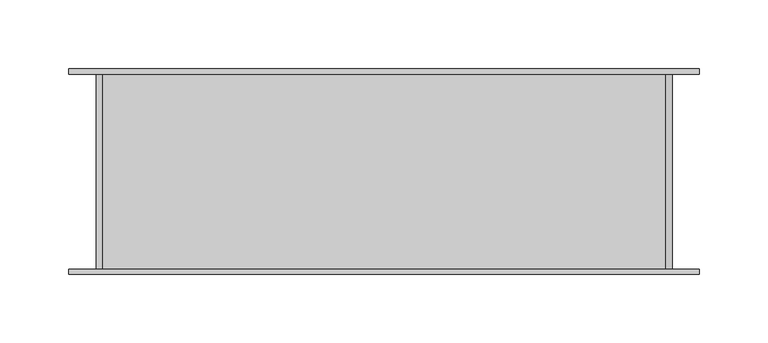
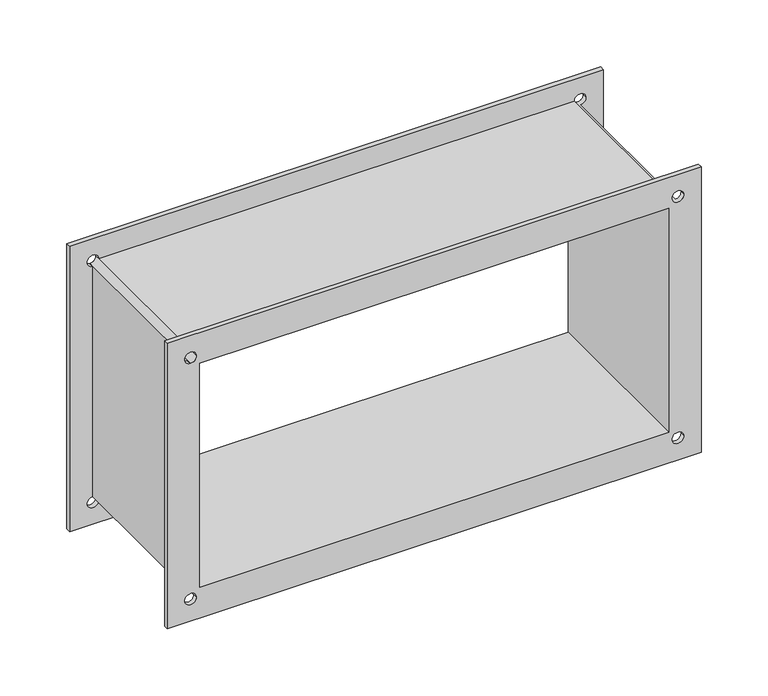
"""IFC4 building model written with IfcOpenShell, lengths in millimetres: proxy geometry, Гибкая вставка В : В 40-20."""

from ifc_helpers import new_model, si_unit, frame, origin, place, context, project, spatial, polyline, circle_curve, source, transform, mapped, element, save
from ifc_brep_helpers import plane_surface, revolved_surface, advanced_brep


def mechanical_equipment_3e9e5508(model_context):
    return source(origin(), model_context, "Body", "AdvancedBrep", [
        advanced_brep(
        [(230.0, 75.0, 130.0), (-230.0, 75.0, 130.0), (-230.0, 70.7949347, 130.0), (230.0, 70.7949347, 130.0), (-230.0, -75.0, 130.0), (230.0, -75.0, 130.0), (230.0, -71.2050653, 130.0), (-230.0, -71.2050653, 130.0), (230.0, -75.0, -130.0), (-230.0, -75.0, -130.0), (-230.0, -71.2050653, -130.0), (230.0, -71.2050653, -130.0), (-230.0, 75.0, -130.0), (230.0, 75.0, -130.0), (230.0, 70.7949347, -130.0), (-230.0, 70.7949347, -130.0), (202.0, 75.0, 102.0), (-202.0, 75.0, 102.0), (-202.0, 75.0, -102.0), (202.0, 75.0, -102.0), (-215.0, 75.0, 110.0), (-205.0, 75.0, 110.0), (205.0, 75.0, 110.0), (215.0, 75.0, 110.0), (205.0, 75.0, -110.0), (215.0, 75.0, -110.0), (-215.0, 75.0, -110.0), (-205.0, 75.0, -110.0), (-202.0, -75.0, 102.0), (202.0, -75.0, 102.0), (202.0, -75.0, -102.0), (-202.0, -75.0, -102.0), (-205.0, -75.0, 110.0), (-215.0, -75.0, 110.0), (215.0, -75.0, 110.0), (205.0, -75.0, 110.0), (215.0, -75.0, -110.0), (205.0, -75.0, -110.0), (-205.0, -75.0, -110.0), (-215.0, -75.0, -110.0), (210.0, 70.7949347, 105.0), (210.0, 70.7949347, -105.0), (215.0, 70.7949347, -110.0), (205.0, 70.7949347, -110.0), (-205.0, 70.7949347, -110.0), (-215.0, 70.7949347, -110.0), (-210.0, 70.7949347, -105.0), (-210.0, 70.7949347, 105.0), (-215.0, 70.7949347, 110.0), (-205.0, 70.7949347, 110.0), (205.0, 70.7949347, 110.0), (215.0, 70.7949347, 110.0), (210.0, -71.2050653, -105.0), (210.0, -71.2050653, 105.0), (215.0, -71.2050653, 110.0), (205.0, -71.2050653, 110.0), (-205.0, -71.2050653, 110.0), (-215.0, -71.2050653, 110.0), (-210.0, -71.2050653, 105.0), (-210.0, -71.2050653, -105.0), (-215.0, -71.2050653, -110.0), (-205.0, -71.2050653, -110.0), (205.0, -71.2050653, -110.0), (215.0, -71.2050653, -110.0)],
        [
            (0, 1),
            (1, 2),
            (2, 3),
            (3, 0),
            (4, 5),
            (5, 6),
            (6, 7),
            (7, 4),
            (8, 9),
            (9, 10),
            (10, 11),
            (11, 8),
            (12, 13),
            (13, 14),
            (14, 15),
            (15, 12),
            (0, 13),
            (12, 1),
            (16, 17),
            (17, 18),
            (18, 19),
            (19, 16),
            (20, 21, circle_curve(frame((-210.0, 75.0, 110.0), z_axis=(0.0, -1.0, 0.0), x_axis=(1.0, 0.0, 0.0)), 5.0)),
            (21, 20, circle_curve(frame((-210.0, 75.0, 110.0), z_axis=(0.0, -1.0, 0.0), x_axis=(1.0, 0.0, 0.0)), 5.0)),
            (22, 23, circle_curve(frame((210.0, 75.0, 110.0), z_axis=(0.0, -1.0, 0.0), x_axis=(1.0, 0.0, 0.0)), 5.0)),
            (23, 22, circle_curve(frame((210.0, 75.0, 110.0), z_axis=(0.0, -1.0, 0.0), x_axis=(1.0, 0.0, 0.0)), 5.0)),
            (24, 25, circle_curve(frame((210.0, 75.0, -110.0), z_axis=(0.0, -1.0, 0.0), x_axis=(1.0, 0.0, 0.0)), 5.0)),
            (25, 24, circle_curve(frame((210.0, 75.0, -110.0), z_axis=(0.0, -1.0, 0.0), x_axis=(1.0, 0.0, 0.0)), 5.0)),
            (26, 27, circle_curve(frame((-210.0, 75.0, -110.0), z_axis=(0.0, -1.0, 0.0), x_axis=(1.0, 0.0, 0.0)), 5.0)),
            (27, 26, circle_curve(frame((-210.0, 75.0, -110.0), z_axis=(0.0, -1.0, 0.0), x_axis=(1.0, 0.0, 0.0)), 5.0)),
            (15, 2),
            (9, 4),
            (7, 10),
            (8, 5),
            (28, 29),
            (29, 30),
            (30, 31),
            (31, 28),
            (32, 33, circle_curve(frame((-210.0, -75.0, 110.0), z_axis=(0.0, 1.0, 0.0), x_axis=(1.0, 0.0, 0.0)), 5.0)),
            (33, 32, circle_curve(frame((-210.0, -75.0, 110.0), z_axis=(0.0, 1.0, 0.0), x_axis=(1.0, 0.0, 0.0)), 5.0)),
            (34, 35, circle_curve(frame((210.0, -75.0, 110.0), z_axis=(0.0, 1.0, 0.0), x_axis=(1.0, 0.0, 0.0)), 5.0)),
            (35, 34, circle_curve(frame((210.0, -75.0, 110.0), z_axis=(0.0, 1.0, 0.0), x_axis=(1.0, 0.0, 0.0)), 5.0)),
            (36, 37, circle_curve(frame((210.0, -75.0, -110.0), z_axis=(0.0, 1.0, 0.0), x_axis=(1.0, 0.0, 0.0)), 5.0)),
            (37, 36, circle_curve(frame((210.0, -75.0, -110.0), z_axis=(0.0, 1.0, 0.0), x_axis=(1.0, 0.0, 0.0)), 5.0)),
            (38, 39, circle_curve(frame((-210.0, -75.0, -110.0), z_axis=(0.0, 1.0, 0.0), x_axis=(1.0, 0.0, 0.0)), 5.0)),
            (39, 38, circle_curve(frame((-210.0, -75.0, -110.0), z_axis=(0.0, 1.0, 0.0), x_axis=(1.0, 0.0, 0.0)), 5.0)),
            (3, 14),
            (11, 6),
            (28, 17),
            (16, 29),
            (31, 18),
            (30, 19),
            (40, 41),
            (41, 42, circle_curve(frame((210.0, 70.7949347, -110.0), z_axis=(0.0, 1.0, 0.0), x_axis=(1.0, 0.0, 0.0)), 5.0)),
            (42, 43, circle_curve(frame((210.0, 70.7949347, -110.0), z_axis=(0.0, 1.0, 0.0), x_axis=(1.0, 0.0, 0.0)), 5.0)),
            (43, 44),
            (44, 45, circle_curve(frame((-210.0, 70.7949347, -110.0), z_axis=(0.0, 1.0, 0.0), x_axis=(1.0, 0.0, 0.0)), 5.0)),
            (45, 46, circle_curve(frame((-210.0, 70.7949347, -110.0), z_axis=(0.0, 1.0, 0.0), x_axis=(1.0, 0.0, 0.0)), 5.0)),
            (46, 47),
            (47, 48, circle_curve(frame((-210.0, 70.7949347, 110.0), z_axis=(0.0, 1.0, 0.0), x_axis=(1.0, 0.0, 0.0)), 5.0)),
            (48, 49, circle_curve(frame((-210.0, 70.7949347, 110.0), z_axis=(0.0, 1.0, 0.0), x_axis=(1.0, 0.0, 0.0)), 5.0)),
            (49, 50),
            (50, 51, circle_curve(frame((210.0, 70.7949347, 110.0), z_axis=(0.0, 1.0, 0.0), x_axis=(1.0, 0.0, 0.0)), 5.0)),
            (51, 40, circle_curve(frame((210.0, 70.7949347, 110.0), z_axis=(0.0, 1.0, 0.0), x_axis=(1.0, 0.0, 0.0)), 5.0)),
            (52, 53),
            (53, 54, circle_curve(frame((210.0, -71.2050653, 110.0), z_axis=(0.0, -1.0, 0.0), x_axis=(1.0, 0.0, 0.0)), 5.0)),
            (54, 55, circle_curve(frame((210.0, -71.2050653, 110.0), z_axis=(0.0, -1.0, 0.0), x_axis=(1.0, 0.0, 0.0)), 5.0)),
            (55, 56),
            (56, 57, circle_curve(frame((-210.0, -71.2050653, 110.0), z_axis=(0.0, -1.0, 0.0), x_axis=(1.0, 0.0, 0.0)), 5.0)),
            (57, 58, circle_curve(frame((-210.0, -71.2050653, 110.0), z_axis=(0.0, -1.0, 0.0), x_axis=(1.0, 0.0, 0.0)), 5.0)),
            (58, 59),
            (59, 60, circle_curve(frame((-210.0, -71.2050653, -110.0), z_axis=(0.0, -1.0, 0.0), x_axis=(1.0, 0.0, 0.0)), 5.0)),
            (60, 61, circle_curve(frame((-210.0, -71.2050653, -110.0), z_axis=(0.0, -1.0, 0.0), x_axis=(1.0, 0.0, 0.0)), 5.0)),
            (61, 62),
            (62, 63, circle_curve(frame((210.0, -71.2050653, -110.0), z_axis=(0.0, -1.0, 0.0), x_axis=(1.0, 0.0, 0.0)), 5.0)),
            (63, 52, circle_curve(frame((210.0, -71.2050653, -110.0), z_axis=(0.0, -1.0, 0.0), x_axis=(1.0, 0.0, 0.0)), 5.0)),
            (32, 56),
            (56, 49),
            (49, 21),
            (20, 48),
            (47, 58),
            (57, 33),
            (55, 35),
            (34, 54),
            (53, 40),
            (51, 23),
            (22, 50),
            (50, 55),
            (62, 37),
            (36, 63),
            (24, 43),
            (42, 25),
            (62, 43),
            (41, 52),
            (38, 61),
            (60, 39),
            (44, 27),
            (26, 45),
            (59, 46),
            (44, 61),
        ],
        [
            plane_surface(frame((-230.0, 75.0, 130.0), z_axis=(0.0, 0.0, 1.0), x_axis=(-1.0, 0.0, 0.0))),
            plane_surface(frame((-230.0, 75.0, -130.0), z_axis=(0.0, 0.0, -1.0), x_axis=(1.0, 0.0, 0.0))),
            plane_surface(frame((230.0, 75.0, 130.0), z_axis=(0.0, 1.0, 0.0), x_axis=(0.0, 0.0, -1.0))),
            plane_surface(frame((-230.0, 75.0, 130.0), z_axis=(-1.0, 0.0, 0.0), x_axis=(0.0, 0.0, -1.0))),
            plane_surface(frame((-230.0, -75.0, 130.0), z_axis=(0.0, -1.0, 0.0), x_axis=(0.0, 0.0, -1.0))),
            plane_surface(frame((230.0, -75.0, 130.0), z_axis=(1.0, 0.0, 0.0), x_axis=(0.0, 0.0, -1.0))),
            plane_surface(frame((202.0, -75.0, 102.0), z_axis=(0.0, 0.0, -1.0), x_axis=(0.0, 1.0, 0.0))),
            plane_surface(frame((-202.0, -75.0, 102.0), z_axis=(1.0, 0.0, 0.0), x_axis=(0.0, 1.0, 0.0))),
            plane_surface(frame((-202.0, -75.0, -102.0), z_axis=(0.0, 0.0, 1.0), x_axis=(0.0, 1.0, 0.0))),
            plane_surface(frame((202.0, -75.0, -102.0), z_axis=(-1.0, 0.0, 0.0), x_axis=(0.0, 1.0, 0.0))),
            plane_surface(frame((-230.0, 70.7949347, 130.0), z_axis=(0.0, -1.0, 0.0), x_axis=(1.0, 0.0, 0.0))),
            plane_surface(frame((-210.0, -71.2050653, 110.0), z_axis=(0.0, 1.0, 0.0), x_axis=(1.0, 0.0, 0.0))),
            revolved_surface(polyline([(-205.0, -75.0, 110.0), (-205.0, 75.0, 110.0)]), (-210.0, 75.0, 110.0), (0.0, -1.0, 0.0)),
            revolved_surface(polyline([(-205.0, -75.0, 110.0), (-205.0, -71.2050653, 110.0)]), (-210.0, 75.0, 110.0), (0.0, -1.0, 0.0)),
            revolved_surface(polyline([(-205.0, 70.7949347, 110.0), (-205.0, 75.0, 110.0)]), (-210.0, 75.0, 110.0), (0.0, -1.0, 0.0)),
            revolved_surface(polyline([(215.0, -75.0, 110.0), (215.0, 75.0, 110.0)]), (210.0, 0.0, 110.0), (0.0, -1.0, 0.0)),
            revolved_surface(polyline([(215.0, -75.0, 110.0), (215.0, -71.2050653, 110.0)]), (210.0, 0.0, 110.0), (0.0, -1.0, 0.0)),
            revolved_surface(polyline([(215.0, 70.7949347, 110.0), (215.0, 75.0, 110.0)]), (210.0, 0.0, 110.0), (0.0, -1.0, 0.0)),
            revolved_surface(polyline([(215.0, -75.0, -110.0), (215.0, -71.2050653, -110.0)]), (210.0, 0.0, -110.0), (0.0, -1.0, 0.0)),
            revolved_surface(polyline([(215.0, 70.7949347, -110.0), (215.0, 75.0, -110.0)]), (210.0, 0.0, -110.0), (0.0, -1.0, 0.0)),
            revolved_surface(polyline([(215.0, -75.0, -110.0), (215.0, 75.0, -110.0)]), (210.0, 0.0, -110.0), (0.0, -1.0, 0.0)),
            revolved_surface(polyline([(-205.0, -75.0, -110.0), (-205.0, -71.2050653, -110.0)]), (-210.0, 0.0, -110.0), (0.0, -1.0, 0.0)),
            revolved_surface(polyline([(-205.0, 70.7949347, -110.0), (-205.0, 75.0, -110.0)]), (-210.0, 0.0, -110.0), (0.0, -1.0, 0.0)),
            revolved_surface(polyline([(-205.0, -75.0, -110.0), (-205.0, 75.0, -110.0)]), (-210.0, 0.0, -110.0), (0.0, -1.0, 0.0)),
            plane_surface(frame((210.0, 70.7949347, 110.0), z_axis=(1.0, 0.0, 0.0), x_axis=(0.0, 0.0, -1.0))),
            plane_surface(frame((210.0, 70.7949347, -110.0), z_axis=(0.0, 0.0, -1.0), x_axis=(-1.0, 0.0, 0.0))),
            plane_surface(frame((-210.0, 70.7949347, -110.0), z_axis=(-1.0, 0.0, 0.0), x_axis=(0.0, 0.0, 1.0))),
            plane_surface(frame((-210.0, 70.7949347, 110.0), z_axis=(0.0, 0.0, 1.0), x_axis=(1.0, 0.0, 0.0))),
        ],
        [
            (0, [[1, 2, 3, 4]]),
            (0, [[5, 6, 7, 8]]),
            (1, [[9, 10, 11, 12]]),
            (1, [[13, 14, 15, 16]]),
            (2, [[-1, 17, -13, 18], [19, 20, 21, 22], [23, 24], [25, 26], [27, 28], [29, 30]]),
            (3, [[-18, -16, 31, -2]]),
            (3, [[32, -8, 33, -10]]),
            (4, [[-5, -32, -9, 34], [35, 36, 37, 38], [39, 40], [41, 42], [43, 44], [45, 46]]),
            (5, [[-17, -4, 47, -14]]),
            (5, [[-34, -12, 48, -6]]),
            (6, [[49, -19, 50, -35]]),
            (7, [[-49, -38, 51, -20]]),
            (8, [[-51, -37, 52, -21]]),
            (9, [[-50, -22, -52, -36]]),
            (10, [[-3, -31, -15, -47], [53, 54, 55, 56, 57, 58, 59, 60, 61, 62, 63, 64]]),
            (11, [[-7, -48, -11, -33], [65, 66, 67, 68, 69, 70, 71, 72, 73, 74, 75, 76]]),
            (12, [[77, 78, 79, -23, 80, -60, 81, -70, 82, -39]]),
            (13, [[-77, -40, -82, -69]]),
            (14, [[-79, -61, -80, -24]]),
            (15, [[83, -41, 84, -66, 85, -64, 86, -25, 87, 88]]),
            (16, [[-83, -67, -84, -42]]),
            (17, [[-87, -26, -86, -63]]),
            (18, [[89, -43, 90, -75]]),
            (19, [[91, -55, 92, -27]]),
            (20, [[-89, 93, -91, -28, -92, -54, 94, -76, -90, -44]]),
            (21, [[95, -73, 96, -45]]),
            (22, [[97, -29, 98, -57]]),
            (23, [[-95, -46, -96, -72, 99, -58, -98, -30, -97, 100]]),
            (24, [[-65, -94, -53, -85]]),
            (25, [[-74, -100, -56, -93]]),
            (26, [[-71, -81, -59, -99]]),
            (27, [[-68, -88, -62, -78]]),
        ],
    ),
    ])


if __name__ == "__main__":
    model = new_model("IFC4")
    model_context = context("Model", 3, world=origin())
    ifc_project = project(units=[si_unit("LENGTHUNIT", "METRE", prefix="MILLI")], contexts=[model_context])
    site = spatial("IfcSite", under=ifc_project)
    building = spatial("IfcBuilding", under=site)
    placement = place(None, origin())
    mechanical_equipment_shape = mechanical_equipment_3e9e5508(model_context)
    element("IfcBuildingElementProxy", 1, Name="Гибкая вставка В : В 40-20", ObjectType="Гибкая вставка В : В 40-20", at=placement, inside=building, context=model_context, shape_type="MappedRepresentation", body=[
        mapped(mechanical_equipment_shape, transform((0.0, 0.0, 0.0), x_axis=(1.0, 0.0, 0.0), y_axis=(0.0, 1.0, 0.0), z_axis=(0.0, 0.0, 1.0))),
    ])
    save(model, "model.ifc")

# Revit data of these elements
# Type "Гибкая вставка В : В 40-20"
#   Manufacturer = "WAER"
#   URL = "https://waer-air.com/"
#   ADSK_Система_Имя [instance default] = ""
#   ADSK_Примечание [instance default] = ""
#   ADSK_Позиция [instance default] = ""
#   ADSK_Обозначение = "В 40-20"
#   ADSK_Наименование = "Гибкая вставка В 40-20"
#   ADSK_Марка = ""
#   ADSK_Код изделия = ""
#   ADSK_Завод-изготовитель = "WAER"
#   ADSK_Единица измерения = "шт."
#   Середина [instance default] = 130 mm
#   Д1 = 130 mm
#   Д = 150 mm
#   Б3 = 200 mm
#   Б2 = 204 mm
#   Б1 = 220 mm
#   А3 = 400 mm
#   А2 = 404 mm
#   А1 = 420 mm
#   А = 460 mm
#   Б = 260 mm
#   ADSK_Расход воздуха = 0 m³/h
#   ADSK_Потеря давления воздуха = 0.0 Pa
#   ADSK_Масса = 1.8
#   Default Elevation = 0
#   Keynote = ""
# Element 1 (IfcBuildingElementProxy, "Гибкая вставка В : В 40-20")
#   Materials on its faces: "Винил_Вент"
# Materials
#   "Винил_Вент": class "Пластик", colour RGB 130 130 130, transparency 0, Description = "Виниловый материал", Cost = 0
